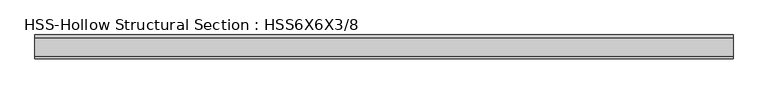
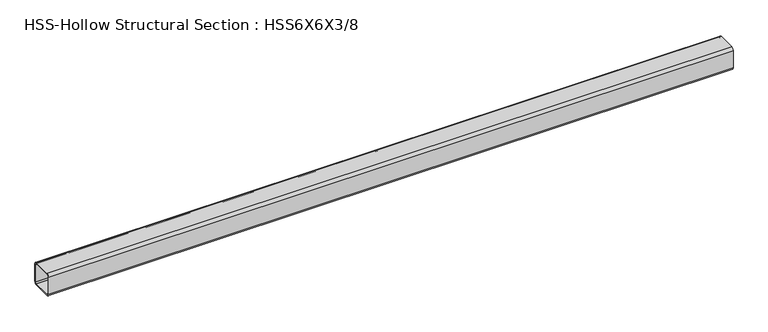
"""IFC4 building model written with IfcOpenShell, lengths in millimetres: member geometry, HSS-Hollow Structural Section : HSS6X6X3/8."""

import ifcopenshell
import ifcopenshell.guid

model = None  # the IFC model being written
_history = None  # IfcOwnerHistory: only IFC2X3 demands one
_inside = {}  # id of a spatial element -> (the spatial element, [elements in it])
_under = {}  # id of a project, library or spatial element -> (it, [spatial elements below it])
_declared = {}  # id of a project -> (the project, [libraries it declares])
_typed = {}  # id of a type object -> (the type object, [elements of that type])
_made_of = {}  # id of a material, layer set ... -> (it, [elements and type objects made of it])


def new_model(schema):
    """Start an empty IFC model of exactly this schema.

    Asked for "IFC4X3", IfcOpenShell would pick the latest addendum, in which some entities
    have other attributes; the version numbers below select the first issue.
    IFC2X3 requires an IfcOwnerHistory on every rooted entity: one is made here for all.
    """
    global model, _history
    if schema == "IFC4X3":
        model = ifcopenshell.file(schema_version=(4, 3, 0, 0))
    else:
        model = ifcopenshell.file(schema=schema)
    _inside.clear()
    _under.clear()
    _declared.clear()
    _typed.clear()
    _made_of.clear()
    _history = None
    if model.schema == "IFC2X3":
        org = make("IfcOrganization", Name="unknown")
        user = make(
            "IfcPersonAndOrganization",
            ThePerson=make("IfcPerson", FamilyName="unknown"),
            TheOrganization=org,
        )
        app = make(
            "IfcApplication",
            ApplicationDeveloper=org,
            Version="unknown",
            ApplicationFullName="unknown",
            ApplicationIdentifier="unknown",
        )
        _history = make(
            "IfcOwnerHistory",
            OwningUser=user,
            OwningApplication=app,
            ChangeAction="ADDED",
            CreationDate=0,
        )
    return model


def make(cls, **values):
    """One entity of the class cls with the attributes given. An attribute that is None is left unset."""
    return model.create_entity(
        cls, **{name: value for name, value in values.items() if value is not None}
    )


def rooted(cls, **values):
    """An entity with a GlobalId (a new one), such as an element, a storey or a relation."""
    return make(cls, GlobalId=ifcopenshell.guid.new(), OwnerHistory=_history, **values)


def si_unit(unit_type, name, prefix=None):
    """IfcSIUnit, for example si_unit("LENGTHUNIT", "METRE", prefix="MILLI")."""
    return make("IfcSIUnit", UnitType=unit_type, Prefix=prefix, Name=name)


def assignment(units):
    """IfcUnitAssignment: the units of a project."""
    return None if units is None else make("IfcUnitAssignment", Units=units)


def point(xyz):
    """IfcCartesianPoint."""
    return None if xyz is None else make("IfcCartesianPoint", Coordinates=xyz)


def direction(xyz):
    """IfcDirection."""
    return None if xyz is None else make("IfcDirection", DirectionRatios=xyz)


def frame(location, z_axis=None, x_axis=None):
    """IfcAxis2Placement3D, a coordinate frame: its origin and axes. An axis left out is left unset."""
    return make(
        "IfcAxis2Placement3D",
        Location=point(location),
        Axis=direction(z_axis),
        RefDirection=direction(x_axis),
    )


def frame_2d(location, x_axis=None):
    """IfcAxis2Placement2D, a coordinate frame in the plane: its origin and x axis."""
    return make(
        "IfcAxis2Placement2D", Location=point(location), RefDirection=direction(x_axis)
    )


def origin():
    """The frame at (0, 0, 0) with its axes left unset."""
    return frame((0.0, 0.0, 0.0))


def place(relative_to, where):
    """IfcLocalPlacement: puts the frame where relative to a parent placement (None: the world)."""
    return make(
        "IfcLocalPlacement", PlacementRelTo=relative_to, RelativePlacement=where
    )


def context(
    kind, dimensions, precision=None, world=None, true_north=None, identifier=None
):
    """IfcGeometricRepresentationContext, for example the 3D "Model" context."""
    return make(
        "IfcGeometricRepresentationContext",
        ContextIdentifier=identifier,
        ContextType=kind,
        CoordinateSpaceDimension=dimensions,
        Precision=precision,
        WorldCoordinateSystem=world,
        TrueNorth=true_north,
    )


def project(units=None, contexts=None):
    """IfcProject with its units and contexts."""
    return rooted(
        "IfcProject",
        Name="project",
        RepresentationContexts=contexts,
        UnitsInContext=assignment(units),
    )


def spatial(cls, under=None, at=None, **own):
    """A site, building, storey or space (cls), placed at a placement, below another one or the project."""
    s = rooted(cls, ObjectPlacement=at, **own)
    if under is not None:
        _under.setdefault(under.id(), (under, []))[1].append(s)
    return s


def polyline(points):
    """IfcPolyline through the points."""
    return make("IfcPolyline", Points=[point(p) for p in points])


def circle_curve(where, radius):
    """IfcCircle in the frame where."""
    return make("IfcCircle", Position=where, Radius=radius)


def trimmed(basis, trim1, trim2, sense, master):
    """IfcTrimmedCurve: the piece of a basis curve between two trims."""
    return make(
        "IfcTrimmedCurve",
        BasisCurve=basis,
        Trim1=trim1,
        Trim2=trim2,
        SenseAgreement=sense,
        MasterRepresentation=master,
    )


def segment(curve, same_sense, transition):
    """IfcCompositeCurveSegment."""
    return make(
        "IfcCompositeCurveSegment",
        Transition=transition,
        SameSense=same_sense,
        ParentCurve=curve,
    )


def composite_curve(segments, self_intersect=None):
    """IfcCompositeCurve: segments joined end to end."""
    return make("IfcCompositeCurve", Segments=segments, SelfIntersect=self_intersect)


def outline(outer, holes=None, kind="AREA"):
    """IfcArbitraryClosedProfileDef: a profile drawn as a closed curve; with holes, ...WithVoids."""
    if holes is None:
        return make("IfcArbitraryClosedProfileDef", ProfileType=kind, OuterCurve=outer)
    return make(
        "IfcArbitraryProfileDefWithVoids",
        ProfileType=kind,
        OuterCurve=outer,
        InnerCurves=holes,
    )


def extrude(swept, where, along, depth):
    """IfcExtrudedAreaSolid: the profile swept, set in the frame where, extruded along a direction by depth."""
    return make(
        "IfcExtrudedAreaSolid",
        SweptArea=swept,
        Position=where,
        ExtrudedDirection=direction(along),
        Depth=depth,
    )


def shape(context_of_items, identifier, shape_type, items):
    """IfcShapeRepresentation: the items that make up one representation, for example the "Body"."""
    return make(
        "IfcShapeRepresentation",
        ContextOfItems=context_of_items,
        RepresentationIdentifier=identifier,
        RepresentationType=shape_type,
        Items=items,
    )


def source(mapping_origin, context_of_items, identifier, shape_type, items):
    """IfcRepresentationMap: a shape defined once, which mapped items show again and again."""
    return make(
        "IfcRepresentationMap",
        MappingOrigin=mapping_origin,
        MappedRepresentation=shape(context_of_items, identifier, shape_type, items),
    )


def transform(
    local_origin,
    x_axis=None,
    y_axis=None,
    z_axis=None,
    scale=None,
    scale2=None,
    scale3=None,
    uniform=True,
):
    """IfcCartesianTransformationOperator3D, or its non-uniform kind. x_axis, y_axis, z_axis: its Axis1, 2, 3."""
    if uniform:
        return make(
            "IfcCartesianTransformationOperator3D",
            Axis1=direction(x_axis),
            Axis2=direction(y_axis),
            LocalOrigin=point(local_origin),
            Scale=scale,
            Axis3=direction(z_axis),
        )
    return make(
        "IfcCartesianTransformationOperator3DnonUniform",
        Axis1=direction(x_axis),
        Axis2=direction(y_axis),
        LocalOrigin=point(local_origin),
        Scale=scale,
        Axis3=direction(z_axis),
        Scale2=scale2,
        Scale3=scale3,
    )


def mapped(mapping_source, mapping_target):
    """IfcMappedItem: shows the shape of a source again, moved by a transform."""
    return make(
        "IfcMappedItem", MappingSource=mapping_source, MappingTarget=mapping_target
    )


def made_of(thing, what):
    """Note that an element or type object is made of a material, layer set ...; save() writes the relation."""
    if what is not None:
        _made_of.setdefault(what.id(), (what, []))[1].append(thing)
    return thing


def element(
    cls,
    number,
    at=None,
    inside=None,
    cuts=None,
    type_object=None,
    material=None,
    context=None,
    identifier="Body",
    shape_type=None,
    held_by="IfcProductDefinitionShape",
    body=None,
    shapes=None,
    **own,
):
    """One element of the class cls, such as IfcWall. Its Tag is "e" and its number.

    at: its placement. inside: the storey or other place that contains it. cuts: it is an
    opening in that element (IfcRelVoidsElement). A single representation is given by context,
    identifier, shape_type and body (its items); several are given by shapes. held_by: the class
    of the entity that holds the representations. save() writes the other relations.
    """
    e = rooted(cls, Tag="e%d" % number, ObjectPlacement=at, **own)
    if body is not None:
        shapes = [shape(context, identifier, shape_type, body)]
    if shapes is not None:
        e.Representation = make(held_by, Representations=shapes)
    if inside is not None:
        _inside.setdefault(inside.id(), (inside, []))[1].append(e)
    if cuts is not None:
        rooted(
            "IfcRelVoidsElement", RelatingBuildingElement=cuts, RelatedOpeningElement=e
        )
    if type_object is not None:
        _typed.setdefault(type_object.id(), (type_object, []))[1].append(e)
    return made_of(e, material)


def aggregate(whole, parts):
    """IfcRelAggregates: a whole, such as a stair, and the parts it consists of."""
    return rooted("IfcRelAggregates", RelatingObject=whole, RelatedObjects=parts)


def save(model, path):
    """Write the relations noted so far, then the file.

    IfcRelAggregates (storeys below a building ...), IfcRelContainedInSpatialStructure (elements
    in a storey), IfcRelDefinesByType, IfcRelAssociatesMaterial and IfcRelDeclares: one each for
    every whole, place, type object, material and project.
    """
    for whole, parts in _under.values():
        aggregate(whole, parts)
    for where, things in _inside.values():
        rooted(
            "IfcRelContainedInSpatialStructure",
            RelatedElements=things,
            RelatingStructure=where,
        )
    for kind, things in _typed.values():
        rooted("IfcRelDefinesByType", RelatedObjects=things, RelatingType=kind)
    for what, things in _made_of.values():
        rooted("IfcRelAssociatesMaterial", RelatedObjects=things, RelatingMaterial=what)
    for by, libraries in _declared.values():
        rooted("IfcRelDeclares", RelatingContext=by, RelatedDefinitions=libraries)
    model.write(path)


def hss_hollow_structural_section_hss6x6x3_8_4cd37dbb(model_context):
    return source(origin(), model_context, "Body", "SweptSolid", [
        extrude(outline(composite_curve([segment(polyline([(76.2, 58.4708), (76.2, -58.4708)]), True, "CONTINUOUS"), segment(trimmed(circle_curve(frame_2d((58.4708, -58.4708)), 17.7292), [point((76.2, -58.4708))], [point((58.4708, -76.2))], False, "CARTESIAN"), True, "CONTINUOUS"), segment(polyline([(58.4708, -76.2), (-58.4708, -76.2)]), True, "CONTINUOUS"), segment(trimmed(circle_curve(frame_2d((-58.4708, -58.4708)), 17.7292), [point((-58.4708, -76.2))], [point((-76.2, -58.4708))], False, "CARTESIAN"), True, "CONTINUOUS"), segment(polyline([(-76.2, -58.4708), (-76.2, 58.4708)]), True, "CONTINUOUS"), segment(trimmed(circle_curve(frame_2d((-58.4708, 58.4708)), 17.7292), [point((-76.2, 58.4708))], [point((-58.4708, 76.2))], False, "CARTESIAN"), True, "CONTINUOUS"), segment(polyline([(-58.4708, 76.2), (58.4708, 76.2)]), True, "CONTINUOUS"), segment(trimmed(circle_curve(frame_2d((58.4708, 58.4708)), 17.7292), [point((58.4708, 76.2))], [point((76.2, 58.4708))], False, "CARTESIAN"), True, "CONTINUOUS")], self_intersect=False), holes=[composite_curve([segment(trimmed(circle_curve(frame_2d((-58.4708, 58.4708)), 8.8646), [point((-58.4708, 67.3354))], [point((-67.3354, 58.4708))], True, "CARTESIAN"), True, "CONTINUOUS"), segment(polyline([(-67.3354, 58.4708), (-67.3354, -58.4708)]), True, "CONTINUOUS"), segment(trimmed(circle_curve(frame_2d((-58.4708, -58.4708)), 8.8646), [point((-67.3354, -58.4708))], [point((-58.4708, -67.3354))], True, "CARTESIAN"), True, "CONTINUOUS"), segment(polyline([(-58.4708, -67.3354), (58.4708, -67.3354)]), True, "CONTINUOUS"), segment(trimmed(circle_curve(frame_2d((58.4708, -58.4708)), 8.8646), [point((58.4708, -67.3354))], [point((67.3354, -58.4708))], True, "CARTESIAN"), True, "CONTINUOUS"), segment(polyline([(67.3354, -58.4708), (67.3354, 58.4708)]), True, "CONTINUOUS"), segment(trimmed(circle_curve(frame_2d((58.4708, 58.4708)), 8.8646), [point((67.3354, 58.4708))], [point((58.4708, 67.3354))], True, "CARTESIAN"), True, "CONTINUOUS"), segment(polyline([(58.4708, 67.3354), (-58.4708, 67.3354)]), True, "CONTINUOUS")], self_intersect=False)]), frame((-2238.0009497, 0.0, 0.0), z_axis=(1.0, 0.0, 0.0), x_axis=(0.0, 1.0, 0.0)), (0.0, 0.0, 1.0), 4449.0151793),
    ])


if __name__ == "__main__":
    model = new_model("IFC4")
    model_context = context("Model", 3, world=origin())
    ifc_project = project(units=[si_unit("LENGTHUNIT", "METRE", prefix="MILLI")], contexts=[model_context])
    site = spatial("IfcSite", under=ifc_project)
    building = spatial("IfcBuilding", under=site)
    placement = place(None, origin())
    hss_hollow_structural_section_hss6x6x3_8_shape = hss_hollow_structural_section_hss6x6x3_8_4cd37dbb(model_context)
    element("IfcMember", 1, ObjectType="HSS-Hollow Structural Section : HSS6X6X3/8", at=placement, inside=building, context=model_context, shape_type="MappedRepresentation", body=[
        mapped(hss_hollow_structural_section_hss6x6x3_8_shape, transform((0.0, 0.0, 0.0), x_axis=(1.0, 0.0, 0.0), y_axis=(0.0, 1.0, 0.0), z_axis=(0.0, 0.0, 1.0))),
    ])
    save(model, "model.ifc")

# Revit data of these elements
# Type "HSS-Hollow Structural Section : HSS6X6X3/8"
#   Assembly Code = "B10"
#   Shape = "Square"
#   W = 27.4
#   Ht = 0' - 6"
#   Length [instance default] = 5' - 0"
#   b = 0' - 6"
#   kr = 0' - 0.698"
#   t = 0' - 0.349"
#   A = 0.0526389 SF
#   Structural Material [instance default] = Steel ASTM A500, Grade B, Rectangular and Square
# Element 1 (IfcMember, "HSS-Hollow Structural Section : HSS6X6X3/8")
#   Materials on its faces: "Steel ASTM A500, Grade B, Rectangular and Square"
# Materials
#   "Steel ASTM A500, Grade B, Rectangular and Square": class "Metal", colour RGB 199 199 199, transparency 0, Description = "Carbon steel", Cost = 0
